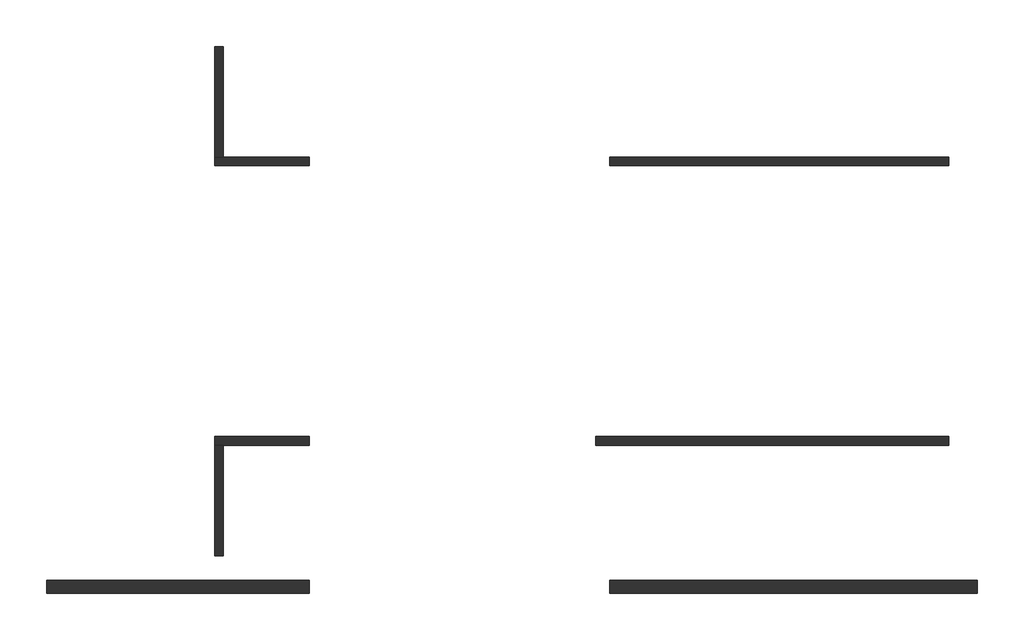
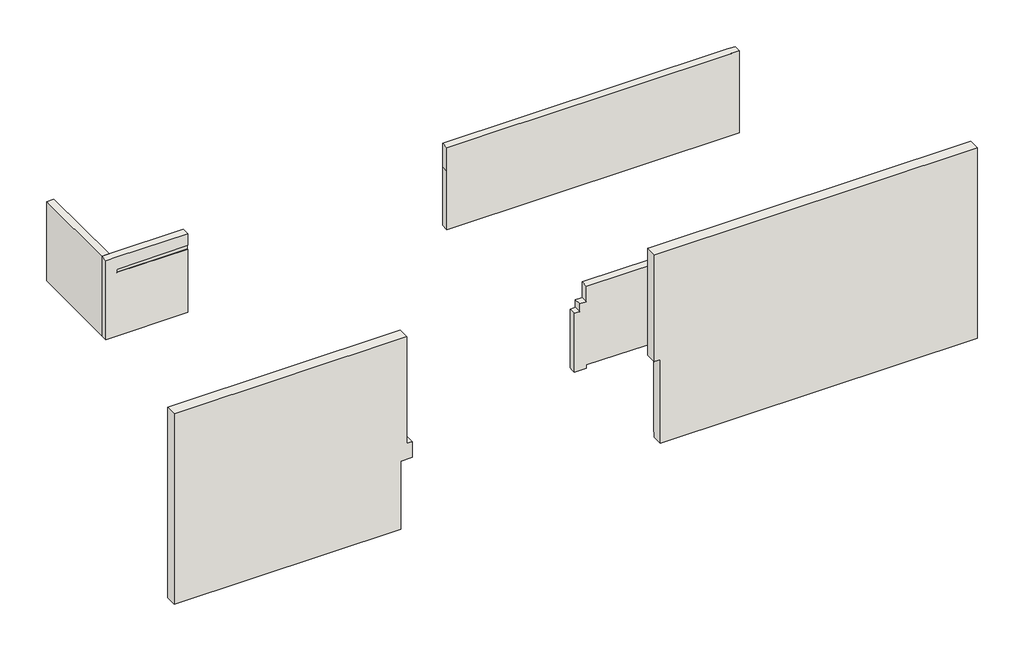
# One storey: 8 walls.
"""IFC4 building model written with IfcOpenShell, lengths in millimetres."""

import ifcopenshell
import ifcopenshell.guid

model = None  # the IFC model being written
_history = None  # IfcOwnerHistory: only IFC2X3 demands one
_inside = {}  # id of a spatial element -> (the spatial element, [elements in it])
_under = {}  # id of a project, library or spatial element -> (it, [spatial elements below it])
_declared = {}  # id of a project -> (the project, [libraries it declares])
_typed = {}  # id of a type object -> (the type object, [elements of that type])
_made_of = {}  # id of a material, layer set ... -> (it, [elements and type objects made of it])


def new_model(schema):
    """Start an empty IFC model of exactly this schema.

    Asked for "IFC4X3", IfcOpenShell would pick the latest addendum, in which some entities
    have other attributes; the version numbers below select the first issue.
    IFC2X3 requires an IfcOwnerHistory on every rooted entity: one is made here for all.
    """
    global model, _history
    if schema == "IFC4X3":
        model = ifcopenshell.file(schema_version=(4, 3, 0, 0))
    else:
        model = ifcopenshell.file(schema=schema)
    _inside.clear()
    _under.clear()
    _declared.clear()
    _typed.clear()
    _made_of.clear()
    _history = None
    if model.schema == "IFC2X3":
        org = make("IfcOrganization", Name="unknown")
        user = make(
            "IfcPersonAndOrganization",
            ThePerson=make("IfcPerson", FamilyName="unknown"),
            TheOrganization=org,
        )
        app = make(
            "IfcApplication",
            ApplicationDeveloper=org,
            Version="unknown",
            ApplicationFullName="unknown",
            ApplicationIdentifier="unknown",
        )
        _history = make(
            "IfcOwnerHistory",
            OwningUser=user,
            OwningApplication=app,
            ChangeAction="ADDED",
            CreationDate=0,
        )
    return model


def make(cls, **values):
    """One entity of the class cls with the attributes given. An attribute that is None is left unset."""
    return model.create_entity(
        cls, **{name: value for name, value in values.items() if value is not None}
    )


def rooted(cls, **values):
    """An entity with a GlobalId (a new one), such as an element, a storey or a relation."""
    return make(cls, GlobalId=ifcopenshell.guid.new(), OwnerHistory=_history, **values)


def si_unit(unit_type, name, prefix=None):
    """IfcSIUnit, for example si_unit("LENGTHUNIT", "METRE", prefix="MILLI")."""
    return make("IfcSIUnit", UnitType=unit_type, Prefix=prefix, Name=name)


def assignment(units):
    """IfcUnitAssignment: the units of a project."""
    return None if units is None else make("IfcUnitAssignment", Units=units)


def point(xyz):
    """IfcCartesianPoint."""
    return None if xyz is None else make("IfcCartesianPoint", Coordinates=xyz)


def direction(xyz):
    """IfcDirection."""
    return None if xyz is None else make("IfcDirection", DirectionRatios=xyz)


def frame(location, z_axis=None, x_axis=None):
    """IfcAxis2Placement3D, a coordinate frame: its origin and axes. An axis left out is left unset."""
    return make(
        "IfcAxis2Placement3D",
        Location=point(location),
        Axis=direction(z_axis),
        RefDirection=direction(x_axis),
    )


def origin():
    """The frame at (0, 0, 0) with its axes left unset."""
    return frame((0.0, 0.0, 0.0))


def place(relative_to, where):
    """IfcLocalPlacement: puts the frame where relative to a parent placement (None: the world)."""
    return make(
        "IfcLocalPlacement", PlacementRelTo=relative_to, RelativePlacement=where
    )


def context(
    kind, dimensions, precision=None, world=None, true_north=None, identifier=None
):
    """IfcGeometricRepresentationContext, for example the 3D "Model" context."""
    return make(
        "IfcGeometricRepresentationContext",
        ContextIdentifier=identifier,
        ContextType=kind,
        CoordinateSpaceDimension=dimensions,
        Precision=precision,
        WorldCoordinateSystem=world,
        TrueNorth=true_north,
    )


def project(units=None, contexts=None):
    """IfcProject with its units and contexts."""
    return rooted(
        "IfcProject",
        Name="project",
        RepresentationContexts=contexts,
        UnitsInContext=assignment(units),
    )


def spatial(cls, under=None, at=None, **own):
    """A site, building, storey or space (cls), placed at a placement, below another one or the project."""
    s = rooted(cls, ObjectPlacement=at, **own)
    if under is not None:
        _under.setdefault(under.id(), (under, []))[1].append(s)
    return s


def polyline(points):
    """IfcPolyline through the points."""
    return make("IfcPolyline", Points=[point(p) for p in points])


def outline(outer, holes=None, kind="AREA"):
    """IfcArbitraryClosedProfileDef: a profile drawn as a closed curve; with holes, ...WithVoids."""
    if holes is None:
        return make("IfcArbitraryClosedProfileDef", ProfileType=kind, OuterCurve=outer)
    return make(
        "IfcArbitraryProfileDefWithVoids",
        ProfileType=kind,
        OuterCurve=outer,
        InnerCurves=holes,
    )


def extrude(swept, where, along, depth):
    """IfcExtrudedAreaSolid: the profile swept, set in the frame where, extruded along a direction by depth."""
    return make(
        "IfcExtrudedAreaSolid",
        SweptArea=swept,
        Position=where,
        ExtrudedDirection=direction(along),
        Depth=depth,
    )


def faces_of(points, faces, orient=None, outer=None):
    """IfcFace entities. A face is a list of loops; a loop is a list of indices into points, from 0.

    orient and outer hold one flag for each loop. By default every Orientation is true, the
    first loop of a face is its IfcFaceOuterBound and the others are IfcFaceBound.
    """
    made = []
    for i, loops in enumerate(faces):
        bounds = []
        for j, loop in enumerate(loops):
            is_outer = j == 0 if outer is None else outer[i][j]
            bounds.append(
                make(
                    "IfcFaceOuterBound" if is_outer else "IfcFaceBound",
                    Bound=make("IfcPolyLoop", Polygon=[points[k] for k in loop]),
                    Orientation=True if orient is None else orient[i][j],
                )
            )
        made.append(make("IfcFace", Bounds=bounds))
    return made


def faceted_brep(points, faces, orient=None, outer=None, voids=None):
    """IfcFacetedBrep: a solid bounded by flat faces; with voids (closed shells), ...WithVoids."""
    shared = [point(p) for p in points]
    hull = make("IfcClosedShell", CfsFaces=faces_of(shared, faces, orient, outer))
    if voids is None:
        return make("IfcFacetedBrep", Outer=hull)
    return make(
        "IfcFacetedBrepWithVoids",
        Outer=hull,
        Voids=[
            make(cls, CfsFaces=faces_of(shared, fs, o, b)) for cls, fs, o, b in voids
        ],
    )


def shape(context_of_items, identifier, shape_type, items):
    """IfcShapeRepresentation: the items that make up one representation, for example the "Body"."""
    return make(
        "IfcShapeRepresentation",
        ContextOfItems=context_of_items,
        RepresentationIdentifier=identifier,
        RepresentationType=shape_type,
        Items=items,
    )


def made_of(thing, what):
    """Note that an element or type object is made of a material, layer set ...; save() writes the relation."""
    if what is not None:
        _made_of.setdefault(what.id(), (what, []))[1].append(thing)
    return thing


def element(
    cls,
    number,
    at=None,
    inside=None,
    cuts=None,
    type_object=None,
    material=None,
    context=None,
    identifier="Body",
    shape_type=None,
    held_by="IfcProductDefinitionShape",
    body=None,
    shapes=None,
    **own,
):
    """One element of the class cls, such as IfcWall. Its Tag is "e" and its number.

    at: its placement. inside: the storey or other place that contains it. cuts: it is an
    opening in that element (IfcRelVoidsElement). A single representation is given by context,
    identifier, shape_type and body (its items); several are given by shapes. held_by: the class
    of the entity that holds the representations. save() writes the other relations.
    """
    e = rooted(cls, Tag="e%d" % number, ObjectPlacement=at, **own)
    if body is not None:
        shapes = [shape(context, identifier, shape_type, body)]
    if shapes is not None:
        e.Representation = make(held_by, Representations=shapes)
    if inside is not None:
        _inside.setdefault(inside.id(), (inside, []))[1].append(e)
    if cuts is not None:
        rooted(
            "IfcRelVoidsElement", RelatingBuildingElement=cuts, RelatedOpeningElement=e
        )
    if type_object is not None:
        _typed.setdefault(type_object.id(), (type_object, []))[1].append(e)
    return made_of(e, material)


def aggregate(whole, parts):
    """IfcRelAggregates: a whole, such as a stair, and the parts it consists of."""
    return rooted("IfcRelAggregates", RelatingObject=whole, RelatedObjects=parts)


def save(model, path):
    """Write the relations noted so far, then the file.

    IfcRelAggregates (storeys below a building ...), IfcRelContainedInSpatialStructure (elements
    in a storey), IfcRelDefinesByType, IfcRelAssociatesMaterial and IfcRelDeclares: one each for
    every whole, place, type object, material and project.
    """
    for whole, parts in _under.values():
        aggregate(whole, parts)
    for where, things in _inside.values():
        rooted(
            "IfcRelContainedInSpatialStructure",
            RelatedElements=things,
            RelatingStructure=where,
        )
    for kind, things in _typed.values():
        rooted("IfcRelDefinesByType", RelatedObjects=things, RelatingType=kind)
    for what, things in _made_of.values():
        rooted("IfcRelAssociatesMaterial", RelatedObjects=things, RelatingMaterial=what)
    for by, libraries in _declared.values():
        rooted("IfcRelDeclares", RelatingContext=by, RelatedDefinitions=libraries)
    model.write(path)


model = new_model("IFC4")

# Units and contexts
model_context = context("Model", 3, world=origin())
ifc_project = project(units=[si_unit("LENGTHUNIT", "METRE", prefix="MILLI")], contexts=[model_context])

# Site, building, storey
site = spatial("IfcSite", under=ifc_project)
building = spatial("IfcBuilding", under=site)
storey = spatial("IfcBuildingStorey", under=building, Name="E-ACCESO", Elevation=-200.0)

# Walls
placement = place(None, origin())
element("IfcWall", 1, ObjectType="MURO TIPO 1_EXTERIOR_PETO_PABLO", at=placement, inside=storey, context=model_context, shape_type="Brep", body=[
    faceted_brep([(-11990.0, -17797.5, 7150.0), (-11975.0, -17797.5, 7150.0), (-205.0, -17797.5, 7150.0), (-205.0, -17797.5, -29.8903052), (-4292.2906333, -17797.5, 0.0), (-8394.5812666, -17797.5, -30.0), (-11770.0, -17797.5, 0.0), (-11770.0, -17797.5, 3030.0), (-11990.0, -17797.5, 3030.0), (-11770.0, -18207.5, -200.0), (-205.0, -18207.5, -200.0), (-205.0, -18207.5, 7150.0), (-11975.0, -18207.5, 7150.0), (-11990.0, -18207.5, 7150.0), (-11990.0, -18207.5, 3030.0), (-11975.0, -18207.5, 3030.0), (-11770.0, -18207.5, 3030.0), (-11770.0, -18207.5, 2430.0), (-11770.0, -17810.0, -200.0), (-205.0, -17810.0, -200.0), (-205.0, -17810.0, -29.8903052), (-8394.5812666, -17810.0, -30.0), (-4292.2906333, -17810.0, 0.0), (-11770.0, -17810.0, 0.0)], [[[0, 1, 2, 3, 4, 5, 6, 7, 8]], [[9, 10, 11, 12, 13, 14, 15, 16, 17]], [[10, 9, 18, 19]], [[2, 1, 0, 13, 12, 11]], [[2, 11, 10, 19, 20, 3]], [[21, 22, 20, 19, 18, 23]], [[20, 22, 4, 3]], [[21, 23, 6, 5]], [[22, 21, 5, 4]], [[13, 0, 8, 14]], [[14, 8, 7, 16, 15]], [[16, 7, 6, 23, 18, 9, 17]]]),
])
element("IfcWall", 2, ObjectType="MURO TIPO 5_PABLO", at=placement, inside=storey, context=model_context, shape_type="Brep", body=[
    faceted_brep([(-24205.0, -13267.5, 3030.0), (-23795.0, -13267.5, 3030.0), (-21230.0, -13267.5, 3030.0), (-20750.0, -13267.5, 3030.0), (-20750.0, -13267.5, 2430.0), (-20790.0, -13267.5, 2430.0), (-21215.0, -13267.5, 2430.0), (-21215.0, -13267.5, 2581.2), (-23795.0, -13267.5, 2551.3734104), (-23810.0, -13267.5, 2551.2), (-23810.0, -13267.5, 2430.0), (-23795.0, -13267.5, 2430.0), (-21230.0, -13267.5, 2430.0), (-21230.0, -13267.5, 0.0), (-24205.0, -13267.5, -28.0660377), (-24205.0, -13267.5, 2130.0), (-20750.0, -13537.5, 3030.0), (-20820.0, -13537.5, 3030.0), (-21230.0, -13537.5, 3030.0), (-23935.0, -13537.5, 3030.0), (-24205.0, -13537.5, 3030.0), (-24205.0, -13537.5, -28.0660377), (-23935.0, -13537.5, -25.5188679), (-21230.0, -13537.5, 0.0), (-21230.0, -13537.5, 2430.0), (-20820.0, -13537.5, 2430.0), (-20750.0, -13537.5, 2430.0), (-23810.0, -13282.5, 2430.0), (-21230.0, -13282.5, 2430.0), (-23810.0, -13282.5, 2551.2), (-21215.0, -13282.5, 2581.2), (-21215.0, -13282.5, 2430.0)], [[[0, 1, 2, 3, 4, 5, 6, 7, 8, 9, 10, 11, 12, 13, 14, 15]], [[16, 17, 18, 19, 20, 21, 22, 23, 24, 25, 26]], [[3, 2, 1, 0, 20, 19, 18, 17, 16]], [[20, 0, 15, 14, 21]], [[27, 28, 12, 11, 10]], [[29, 27, 10, 9]], [[27, 29, 30, 31, 28]], [[30, 29, 9, 8, 7]], [[14, 13, 23, 22, 21]], [[26, 25, 24, 28, 31, 6, 5, 4]], [[13, 12, 28, 24, 23]], [[4, 3, 16, 26]], [[31, 30, 7, 6]]]),
])
element("IfcWall", 3, ObjectType="MURO TIPO 5_PABLO", at=placement, inside=storey, context=model_context, shape_type="SweptSolid", body=[
    extrude(outline(polyline([(3030.0, -23935.0), (3030.0, -24205.0), (-28.0660377, -24205.0), (-25.5188679, -23935.0), (3030.0, -23935.0)])), frame((0.0, -17017.5, 0.0), z_axis=(0.0, 1.0, 0.0), x_axis=(0.0, 0.0, 1.0)), (0.0, 0.0, 1.0), 3480.0),
])
element("IfcWall", 4, ObjectType="MURO TIPO 5_PETO CUB_PABLO", at=placement, inside=storey, context=model_context, shape_type="Brep", body=[
    faceted_brep([(-1110.0, -13537.5, -23.2720515), (-1110.0, -13537.5, 3030.0), (-1380.0, -13537.5, 3030.0), (-1395.1532376, -13537.5, 3030.0), (-1410.1532376, -13537.5, 3030.0), (-1425.0, -13537.5, 3030.0), (-8795.0, -13537.5, 3030.0), (-9065.0, -13537.5, 3030.0), (-11770.0, -13537.5, 3030.0), (-11770.0, -13537.5, 2430.0), (-12010.0, -13537.5, 2430.0), (-12010.0, -13537.5, 2130.0), (-12210.0, -13537.5, 2130.0), (-12210.0, -13537.5, -135.0), (-11770.0, -13537.5, -135.0), (-11770.0, -13537.5, 0.0), (-9065.0, -13537.5, -24.0414616), (-8795.0, -13537.5, -26.4411639), (-8394.5812666, -13537.5, -30.0), (-4292.2906333, -13537.5, 0.0), (-1380.0, -13537.5, -21.2975449), (-1110.0, -13267.5, 3030.0), (-1110.0, -13267.5, -23.2720515), (-4292.2906333, -13267.5, 0.0), (-8394.5812666, -13267.5, -30.0), (-11770.0, -13267.5, 0.0), (-11770.0, -13267.5, -135.0), (-12210.0, -13267.5, -135.0), (-12210.0, -13267.5, 2100.0), (-12210.0, -13267.5, 2130.0), (-12010.0, -13267.5, 2130.0), (-12010.0, -13267.5, 2430.0), (-11785.0, -13267.5, 2430.0), (-11770.0, -13267.5, 2430.0), (-11770.0, -13267.5, 3030.0), (-9205.0, -13267.5, 3030.0), (-8795.0, -13267.5, 3030.0), (-1425.0, -13267.5, 3030.0), (-1410.1532376, -13267.5, 3030.0), (-1395.1532376, -13267.5, 3030.0), (-1380.0, -13267.5, 3030.0), (-12210.0, -13372.5, -135.0)], [[[0, 1, 2, 3, 4, 5, 6, 7, 8, 9, 10, 11, 12, 13, 14, 15, 16, 17, 18, 19, 20]], [[21, 22, 23, 24, 25, 26, 27, 28, 29, 30, 31, 32, 33, 34, 35, 36, 37, 38, 39, 40]], [[26, 14, 13, 41, 27]], [[1, 21, 40, 39, 38, 37, 36, 35, 34, 8, 7, 6, 5, 4, 3, 2]], [[21, 1, 0, 22]], [[0, 20, 19, 23, 22]], [[24, 18, 17, 16, 15, 25]], [[18, 24, 23, 19]], [[25, 15, 14, 26]], [[11, 30, 29, 12]], [[30, 11, 10, 31]], [[33, 32, 31, 10, 9]], [[27, 41, 13, 12, 29, 28]], [[8, 34, 33, 9]]]),
])
element("IfcWall", 5, ObjectType="MURO TIPO 5_PABLO", at=placement, inside=storey, context=model_context, shape_type="Brep", body=[
    faceted_brep([(-24205.0, -4462.5, 3030.0), (-23935.0, -4462.5, 3030.0), (-21230.0, -4462.5, 3030.0), (-21230.0, -4462.5, 0.0), (-23935.0, -4462.5, -25.5188679), (-24205.0, -4462.5, -28.0660377), (-21230.0, -4732.5, 3030.0), (-23795.0, -4732.5, 3030.0), (-24205.0, -4732.5, 3030.0), (-24205.0, -4732.5, 2130.0), (-24205.0, -4732.5, -28.0660377), (-21230.0, -4732.5, 0.0), (-21230.0, -4732.5, 2430.0), (-23795.0, -4732.5, 2430.0), (-23810.0, -4732.5, 2430.0), (-23810.0, -4732.5, 2551.2), (-23795.0, -4732.5, 2551.3734104), (-21230.0, -4732.5, 2581.0265896), (-21230.0, -4717.5, 2581.0265896), (-21230.0, -4717.5, 2430.0), (-23810.0, -4717.5, 2430.0), (-23810.0, -4717.5, 2551.2)], [[[0, 1, 2, 3, 4, 5]], [[6, 7, 8, 9, 10, 11, 12, 13, 14, 15, 16, 17]], [[2, 1, 0, 8, 7, 6]], [[2, 6, 17, 18, 19, 12, 11, 3]], [[8, 0, 5, 10, 9]], [[20, 14, 13, 12, 19]], [[21, 20, 19, 18]], [[20, 21, 15, 14]], [[21, 18, 17, 16, 15]], [[5, 4, 3, 11, 10]]]),
])
element("IfcWall", 6, ObjectType="MURO TIPO 5_PABLO", at=placement, inside=storey, context=model_context, shape_type="SweptSolid", body=[
    extrude(outline(polyline([(3030.0, -23935.0), (3030.0, -24205.0), (-28.0660377, -24205.0), (-25.5188679, -23935.0), (3030.0, -23935.0)])), frame((0.0, -4462.5, 0.0), z_axis=(0.0, 1.0, 0.0), x_axis=(0.0, 0.0, 1.0)), (0.0, 0.0, 1.0), 3480.0),
])
element("IfcWall", 7, ObjectType="MURO TIPO 5_PETO CUB_PABLO", at=placement, inside=storey, context=model_context, shape_type="Brep", body=[
    faceted_brep([(-11770.0, -4732.5, -135.0), (-1110.0, -4732.5, -135.0), (-1110.0, -4732.5, 3030.0), (-1380.0, -4732.5, 3030.0), (-1395.1532376, -4732.5, 3030.0), (-1410.1532376, -4732.5, 3030.0), (-1425.0, -4732.5, 3030.0), (-8795.0, -4732.5, 3030.0), (-9205.0, -4732.5, 3030.0), (-11770.0, -4732.5, 3030.0), (-11770.0, -4732.5, 2130.0), (-11770.0, -4732.5, 2100.0), (-11770.0, -4732.5, 0.0), (-1110.0, -4462.5, -135.0), (-11770.0, -4462.5, -135.0), (-11770.0, -4462.5, 2100.0), (-11770.0, -4462.5, 3030.0), (-9065.0, -4462.5, 3030.0), (-8795.0, -4462.5, 3030.0), (-1425.0, -4462.5, 3030.0), (-1410.1532376, -4462.5, 3030.0), (-1395.1532376, -4462.5, 3030.0), (-1380.0, -4462.5, 3030.0), (-1110.0, -4462.5, 3030.0), (-1110.0, -4462.5, -23.2720515)], [[[0, 1, 2, 3, 4, 5, 6, 7, 8, 9, 10, 11, 12]], [[13, 14, 15, 16, 17, 18, 19, 20, 21, 22, 23, 24]], [[1, 0, 14, 13]], [[2, 23, 22, 21, 20, 19, 18, 17, 16, 9, 8, 7, 6, 5, 4, 3]], [[2, 1, 13, 24, 23]], [[0, 12, 11, 15, 14]], [[9, 16, 15, 11, 10]]]),
])
element("IfcWall", 8, ObjectType="MURO TIPO 1_EXTERIOR_PETO_PABLO", at=placement, inside=storey, context=model_context, shape_type="Brep", body=[
    faceted_brep([(-21230.0, -17797.5, -200.0), (-29500.0, -17797.5, -200.0), (-29500.0, -17797.5, 0.0), (-29500.0, -17797.5, 7150.0), (-21025.0, -17797.5, 7150.0), (-21010.0, -17797.5, 7150.0), (-21010.0, -17797.5, 3030.0), (-20820.0, -17797.5, 3030.0), (-20820.0, -17797.5, 2921.0618785), (-20820.0, -17797.5, 2730.0), (-20820.0, -17797.5, 2430.0), (-21230.0, -17797.5, 2430.0), (-29500.0, -18207.5, -200.0), (-21230.0, -18207.5, -200.0), (-21230.0, -18207.5, 2430.0), (-20820.0, -18207.5, 2430.0), (-20820.0, -18207.5, 3030.0), (-21010.0, -18207.5, 3030.0), (-21010.0, -18207.5, 7150.0), (-21025.0, -18207.5, 7150.0), (-29500.0, -18207.5, 7150.0), (-29500.0, -18207.5, 0.0)], [[[0, 1, 2, 3, 4, 5, 6, 7, 8, 9, 10, 11]], [[12, 13, 14, 15, 16, 17, 18, 19, 20, 21]], [[1, 0, 13, 12]], [[3, 2, 1, 12, 21, 20]], [[5, 4, 3, 20, 19, 18]], [[5, 18, 17, 6]], [[0, 11, 14, 13]], [[10, 9, 8, 7, 16, 15]], [[15, 14, 11, 10]], [[6, 17, 16, 7]]]),
])

save(model, "model.ifc")

# Revit data of these elements
# Project information
#   Fecha de emisión de proyecto = "Fecha de emisión"
#   Estado de proyecto = "Estado de proyecto"
#   Nombre de cliente = "Propietario"
#   Dirección de proyecto = "Introduzca dirección aquí"
#   Nombre de proyecto = "Nombre de proyecto"
#   Número de proyecto = "0001"
# Grids (mm)
#   "10": line (-29500, 9189.325) -> (-29500, -29213.653)
#   "1": line (-33000, 9189.325) -> (-33000, -29213.653)
#   "B": line (7688.401, -13500) -> (-37134.551, -13500)
#   "A": line (7688.401, -18000) -> (-37134.551, -18000)
#   "BC": line (7688.401, -9000) -> (-37134.551, -9000)
#   "C": line (7688.401, -4500) -> (-37134.551, -4500)
#   "D": line (7688.401, 0) -> (-37134.551, 0)
#   "6": line (0, 9189.325) -> (0, -29213.653)
#   "56": line (-6000, 9189.325) -> (-6000, -29213.653)
#   "5": line (-9000, 9189.325) -> (-9000, -29213.653)
#   "4": line (-12000, 9189.325) -> (-12000, -29213.653)
#   "3": line (-21000, 9189.325) -> (-21000, -29213.653)
#   "2": line (-24000, 9189.325) -> (-24000, -29213.653)
#   "12": line (-27000, 9189.325) -> (-27000, -29213.653)
# Type "MURO TIPO 1_EXTERIOR_PETO_PABLO"
#   Keynote = "Md.1"
#   Description = "Muro interior-exterior perimetral"
#   Type Mark = "M1"
#   Layers, outside or top first: 0.015 m "Enfoscado cemento y pintura" (function 5); 0.115 m "Ladrillo cerámico perforado" (function 1); 0.15 m "Aire" (function 3); 0.115 m "Ladrillo cerámico perforado" (function 1); 0.015 m "Enfoscado cemento y pintura" (function 5)
# Type "MURO TIPO 5_PABLO"
#   Keynote = "Md.1"
#   Description = "Muro interior-interior patio exterior"
#   Type Mark = "M5"
#   Layers, outside or top first: 0.015 m "Enfoscado cemento y pintura" (function 5); 0.24 m "Ladrillo cerámico perforado" (function 1); 0.015 m "Enfoscado cemento y pintura" (function 5)
# Type "MURO TIPO 5_PETO CUB_PABLO"
#   Keynote = "Md.1"
#   Description = "Muro interior-interior patio exterior"
#   Type Mark = "M5"
#   Layers, outside or top first: 0.015 m "Enfoscado cemento y pintura" (function 5); 0.24 m "Ladrillo cerámico perforado" (function 1); 0.015 m "Enfoscado cemento y pintura" (function 5)
# Elements 1, 8 (IfcWall, "MURO TIPO 1_EXTERIOR_PETO_PABLO")
#   Top Offset = 0.00 m
#   Base Offset = 0.00 m
#   wall height = 7.35 m
#   Phase Created = Nueva construcción
#   Base Constraint = E-ACCESO
#   Top Constraint = AUXILIAR-CoronacionMuro
#   Materials on its faces: "Muro por defecto", "Enfoscado cemento y pintura"
# Element 2 (IfcWall, "MURO TIPO 5_PABLO")
#   built-in parameter 1001111 = 0.065 m
#   Top Offset = 0.00 m
#   Base Offset = 0.065 m
#   wall height = 3.165 m
#   Phase Created = Nueva construcción
#   Base Constraint = E-ACCESO
#   Top Constraint = AUXILIAR-Peto
#   Materials on its faces: "Muro por defecto", "Enfoscado cemento y pintura", "Enlucido de yeso"
# Elements 3, 5, 6 (IfcWall, "MURO TIPO 5_PABLO")
#   built-in parameter 1001111 = 0.065 m
#   Top Offset = 0.00 m
#   Base Offset = 0.065 m
#   wall height = 3.165 m
#   Phase Created = Nueva construcción
#   Base Constraint = E-ACCESO
#   Top Constraint = AUXILIAR-Peto
#   Materials on its faces: "Muro por defecto", "Enfoscado cemento y pintura"
# Element 4 (IfcWall, "MURO TIPO 5_PETO CUB_PABLO")
#   built-in parameter 1001111 = 0.065 m
#   Top Offset = 0.00 m
#   Base Offset = 0.065 m
#   wall height = 3.165 m
#   Phase Created = Nueva construcción
#   Base Constraint = E-ACCESO
#   Top Constraint = AUXILIAR-Peto
#   Materials on its faces: "Muro por defecto", "Enfoscado cemento y pintura", "Enlucido de yeso"
# Element 7 (IfcWall, "MURO TIPO 5_PETO CUB_PABLO")
#   built-in parameter 1001111 = 0.065 m
#   Top Offset = 0.00 m
#   Base Offset = 0.065 m
#   wall height = 3.165 m
#   Phase Created = Nueva construcción
#   Base Constraint = E-ACCESO
#   Top Constraint = AUXILIAR-Peto
#   Materials on its faces: "Muro por defecto", "Enfoscado cemento y pintura"
# Materials
#   "Enfoscado cemento y pintura": class "Varios", colour RGB 127 127 127, transparency 0, Keynote = "2", Comments = "Color blanco (1,5 cm)", Cost = 0
#   "Ladrillo cerámico perforado": class "Enladrillado", colour RGB 204 146 111, transparency 0, Cost = 0
#   "Aire": class "Gas", colour RGB 183 255 255, transparency 0.75, Description = "Aire", Cost = 0
#   "Muro por defecto": class "Varios", colour RGB 212 212 212, transparency 0, Cost = 0
#   "Enlucido de yeso": class "Placa de yeso laminado", colour RGB 249 249 249, transparency 0, Keynote = "1", Comments = "Color blanco al temple (1,5 cm)", Description = "1", Cost = 0
